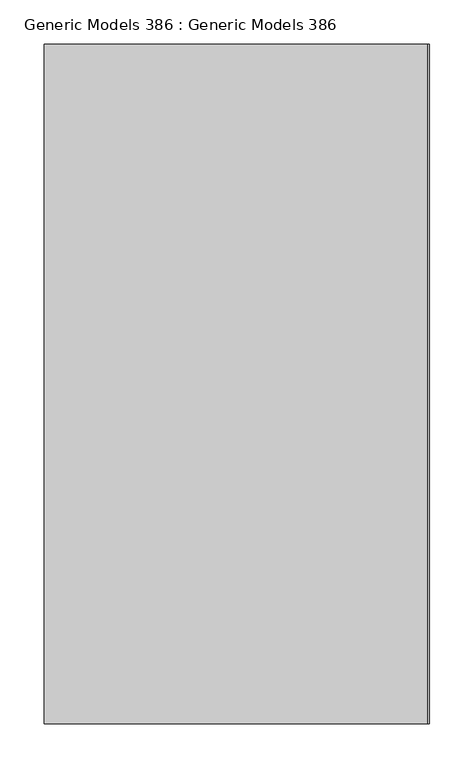
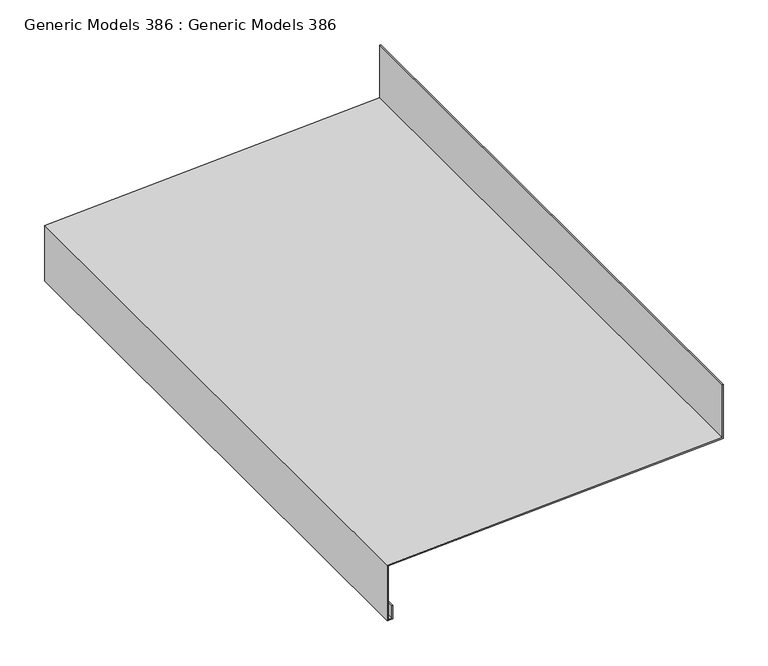
"""IFC4 building model written with IfcOpenShell, lengths in millimetres: proxy geometry, Generic Models 386 : Generic Models 386."""

from ifc_helpers import new_model, si_unit, frame, origin, place, context, project, spatial, polyline, outline, extrude, source, transform, mapped, element, save


def generic_models_386_generic_models_386_06e2602e(model_context):
    return source(origin(), model_context, "Body", "SweptSolid", [
        extrude(outline(polyline([(129140.7263161, -6632.5659398), (129213.9030995, -6632.5659398), (129213.9030995, -6633.8557835), (129141.9503321, -6633.8557835), (129119.3164639, -7065.7357168), (129043.2944712, -7065.7357168), (129043.2944712, -7058.0866564), (129061.7628835, -7058.0866564), (129061.7628835, -7059.3765001), (129044.6740495, -7059.3765001), (129044.6740495, -7064.445873), (129118.0924479, -7064.445873), (129140.7263161, -6632.5659398)])), frame((0.0, -4250.542257, 0.0), z_axis=(0.0, 1.0, 0.0), x_axis=(0.0, 0.0, 1.0)), (0.0, 0.0, 1.0), 763.8192232),
    ])


if __name__ == "__main__":
    model = new_model("IFC4")
    model_context = context("Model", 3, world=origin())
    ifc_project = project(units=[si_unit("LENGTHUNIT", "METRE", prefix="MILLI")], contexts=[model_context])
    site = spatial("IfcSite", under=ifc_project)
    building = spatial("IfcBuilding", under=site)
    placement = place(None, origin())
    generic_models_386_generic_models_386_shape = generic_models_386_generic_models_386_06e2602e(model_context)
    element("IfcBuildingElementProxy", 1, Name="Generic Models 386 : Generic Models 386", ObjectType="Generic Models 386 : Generic Models 386", at=placement, inside=building, context=model_context, shape_type="MappedRepresentation", body=[
        mapped(generic_models_386_generic_models_386_shape, transform((0.0, 0.0, 0.0), x_axis=(1.0, 0.0, 0.0), y_axis=(0.0, 1.0, 0.0), z_axis=(0.0, 0.0, 1.0))),
    ])
    save(model, "model.ifc")

# Revit data of these elements
# Element 1 (IfcBuildingElementProxy, "Generic Models 386 : Generic Models 386")
#   Materials on its faces: "_16 GA. COPPER BRAKE METAL FASCIA"
# Materials
#   "_16 GA. COPPER BRAKE METAL FASCIA": class "Generic", colour RGB 175 175 175, transparency 0, Cost = 0
